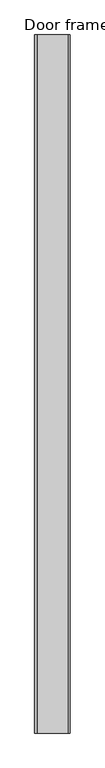
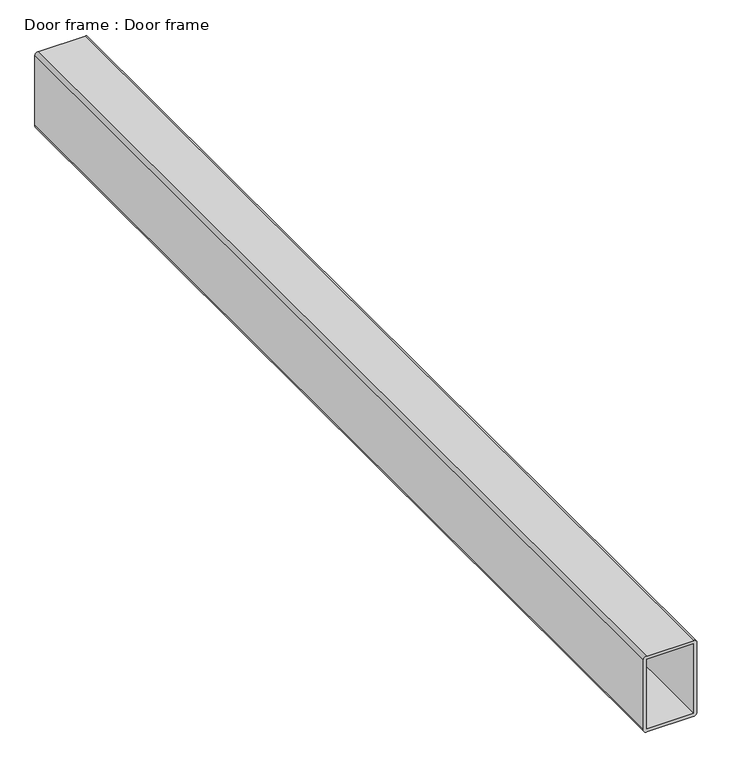
"""IFC4 building model written with IfcOpenShell, lengths in millimetres: proxy geometry, Door frame : Door frame."""

from ifc_helpers import new_model, si_unit, point, frame, frame_2d, origin, place, context, project, spatial, polyline, circle_curve, trimmed, segment, composite_curve, outline, extrude, source, transform, mapped, element, save


def door_frame_door_frame_b90efb81(model_context):
    return source(origin(), model_context, "Body", "SweptSolid", [
        extrude(outline(composite_curve([segment(polyline([(34855.8775473, -8390.3106967), (34855.8775473, -8301.4106967)]), True, "CONTINUOUS"), segment(trimmed(circle_curve(frame_2d((34862.2275473, -8301.4106967)), 6.35), [point((34855.8775473, -8301.4106967))], [point((34862.2275473, -8295.0606967))], False, "CARTESIAN"), True, "CONTINUOUS"), segment(polyline([(34862.2275473, -8295.0606967), (35001.9275473, -8295.0606967)]), True, "CONTINUOUS"), segment(trimmed(circle_curve(frame_2d((35001.9275473, -8301.4106967)), 6.35), [point((35001.9275473, -8295.0606967))], [point((35008.2775473, -8301.4106967))], False, "CARTESIAN"), True, "CONTINUOUS"), segment(polyline([(35008.2775473, -8301.4106967), (35008.2775473, -8390.3106967)]), True, "CONTINUOUS"), segment(trimmed(circle_curve(frame_2d((35001.9275473, -8390.3106967)), 6.35), [point((35008.2775473, -8390.3106967))], [point((35001.9275473, -8396.6606967))], False, "CARTESIAN"), True, "CONTINUOUS"), segment(polyline([(35001.9275473, -8396.6606967), (34862.2275473, -8396.6606967)]), True, "CONTINUOUS"), segment(trimmed(circle_curve(frame_2d((34862.2275473, -8390.3106967)), 6.35), [point((34862.2275473, -8396.6606967))], [point((34855.8775473, -8390.3106967))], False, "CARTESIAN"), True, "CONTINUOUS")], self_intersect=False), holes=[polyline([(35001.7775473, -8301.5606967), (34862.3775473, -8301.5606967), (34862.3775473, -8390.1606967), (35001.7775473, -8390.1606967), (35001.7775473, -8301.5606967)])]), frame((0.0, 4540.4513244, 0.0), z_axis=(0.0, 1.0, 0.0), x_axis=(0.0, 0.0, 1.0)), (0.0, 0.0, 1.0), 2000.0),
    ])


if __name__ == "__main__":
    model = new_model("IFC4")
    model_context = context("Model", 3, world=origin())
    ifc_project = project(units=[si_unit("LENGTHUNIT", "METRE", prefix="MILLI")], contexts=[model_context])
    site = spatial("IfcSite", under=ifc_project)
    building = spatial("IfcBuilding", under=site)
    placement = place(None, origin())
    door_frame_door_frame_shape = door_frame_door_frame_b90efb81(model_context)
    element("IfcBuildingElementProxy", 1, Name="Door frame : Door frame", ObjectType="Door frame : Door frame", at=placement, inside=building, context=model_context, shape_type="MappedRepresentation", body=[
        mapped(door_frame_door_frame_shape, transform((0.0, 0.0, 0.0), x_axis=(1.0, 0.0, 0.0), y_axis=(0.0, 1.0, 0.0), z_axis=(0.0, 0.0, 1.0))),
    ])
    save(model, "model.ifc")

# Revit data of these elements
# Type "Door frame : Door frame"
#   NameOverride = "Door frame"
# Element 1 (IfcBuildingElementProxy, "Door frame : Door frame")
#   Materials on its faces: "DOOR FRAME: TUBE STEEL PROFILE - METALIZED, PRIMED & PAINTED (COLOR PER ARCHITECT)"
# Materials
#   "DOOR FRAME: TUBE STEEL PROFILE - METALIZED, PRIMED & PAINTED (COLOR PER ARCHITECT)": class "Unassigned", colour RGB 128 128 128, transparency 0, Cost = 0
